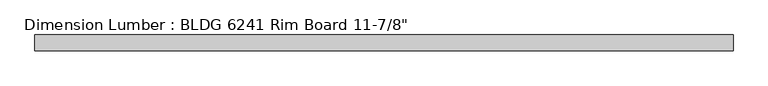
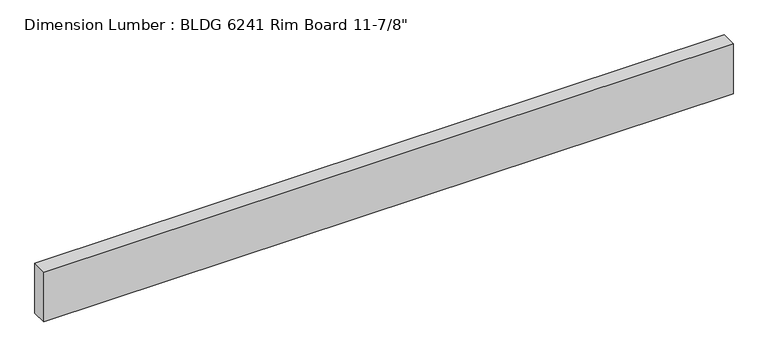
"""IFC4 building model written with IfcOpenShell, lengths in millimetres: beam geometry."""

from ifc_helpers import new_model, si_unit, frame, origin, place, context, project, spatial, polyline, outline, extrude, source, transform, mapped, element, save


def beam_dcf2d3fa(model_context):
    return source(origin(), model_context, "Body", "SweptSolid", [
        extrude(outline(polyline([(1927.225, 44.45), (1927.225, -44.45), (-2016.125, -44.45), (-2016.125, 44.45), (1927.225, 44.45)])), frame((0.0, 0.0, -150.8125), z_axis=(0.0, 0.0, 1.0), x_axis=(1.0, 0.0, 0.0)), (0.0, 0.0, 1.0), 301.625),
    ])


if __name__ == "__main__":
    model = new_model("IFC4")
    model_context = context("Model", 3, world=origin())
    ifc_project = project(units=[si_unit("LENGTHUNIT", "METRE", prefix="MILLI")], contexts=[model_context])
    site = spatial("IfcSite", under=ifc_project)
    building = spatial("IfcBuilding", under=site)
    placement = place(None, origin())
    beam_shape = beam_dcf2d3fa(model_context)
    element("IfcBeam", 1, ObjectType="Dimension Lumber : BLDG 6241 Rim Board 11-7/8\"", at=placement, inside=building, context=model_context, shape_type="MappedRepresentation", body=[
        mapped(beam_shape, transform((0.0, 0.0, 0.0), x_axis=(1.0, 0.0, 0.0), y_axis=(0.0, 1.0, 0.0), z_axis=(0.0, 0.0, 1.0))),
    ])
    save(model, "model.ifc")

# Revit data of these elements
# Type "Dimension Lumber : BLDG 6241 Rim Board 11-7/8\""
#   Assembly Code = "B10"
#   A = 0.273472 SF
#   Length [instance default] = 5' - 0"
#   b = 0' - 3 1/2"
#   d = 0' - 11 7/8"
#   Structural Material [instance default] = Softwood, Lumber
# Element 1 (IfcBeam, "Dimension Lumber : BLDG 6241 Rim Board 11-7/8\"")
#   Materials on its faces: "Softwood, Lumber"
# Materials
#   "Softwood, Lumber": class "Wood", colour RGB 223 192 134, transparency 0, Description = "Pinus Echinata", Cost = 0
